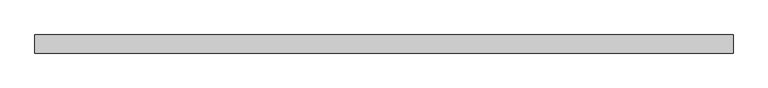
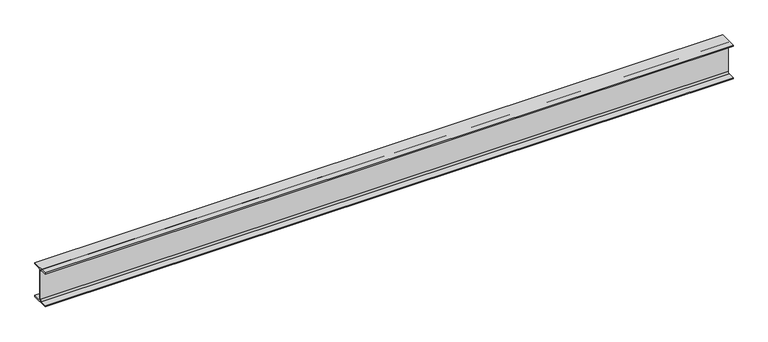
"""IFC4 building model written with IfcOpenShell, lengths in millimetres: beam geometry, 0912_Steel Framing_H-KSD3502 : H_SB_ASB_H-250x125x6x9."""

from ifc_helpers import new_model, si_unit, point, frame, frame_2d, origin, place, context, project, spatial, polyline, circle_curve, trimmed, segment, composite_curve, outline, extrude, source, transform, mapped, element, save


def beam_1a29c797(model_context):
    return source(origin(), model_context, "Body", "SweptSolid", [
        extrude(outline(composite_curve([segment(polyline([(62.5, -116.0), (62.5, -125.0), (-62.5, -125.0), (-62.5, -116.0), (-15.0, -116.0)]), True, "CONTINUOUS"), segment(trimmed(circle_curve(frame_2d((-15.0, -104.0)), 12.0), [point((-15.0, -116.0))], [point((-3.0, -104.0))], True, "CARTESIAN"), True, "CONTINUOUS"), segment(polyline([(-3.0, -104.0), (-3.0, 104.0)]), True, "CONTINUOUS"), segment(trimmed(circle_curve(frame_2d((-15.0, 104.0)), 12.0), [point((-3.0, 104.0))], [point((-15.0, 116.0))], True, "CARTESIAN"), True, "CONTINUOUS"), segment(polyline([(-15.0, 116.0), (-62.5, 116.0), (-62.5, 125.0), (62.5, 125.0), (62.5, 116.0), (15.0, 116.0)]), True, "CONTINUOUS"), segment(trimmed(circle_curve(frame_2d((15.0, 104.0)), 12.0), [point((15.0, 116.0))], [point((3.0, 104.0))], True, "CARTESIAN"), True, "CONTINUOUS"), segment(polyline([(3.0, 104.0), (3.0, -104.0)]), True, "CONTINUOUS"), segment(trimmed(circle_curve(frame_2d((15.0, -104.0)), 12.0), [point((3.0, -104.0))], [point((15.0, -116.0))], True, "CARTESIAN"), True, "CONTINUOUS"), segment(polyline([(15.0, -116.0), (62.5, -116.0)]), True, "CONTINUOUS")], self_intersect=False)), frame((-2404.8281705, 0.0, 0.0), z_axis=(1.0, 0.0, 0.0), x_axis=(0.0, 1.0, 0.0)), (0.0, 0.0, 1.0), 4808.1916513),
    ])


if __name__ == "__main__":
    model = new_model("IFC4")
    model_context = context("Model", 3, world=origin())
    ifc_project = project(units=[si_unit("LENGTHUNIT", "METRE", prefix="MILLI")], contexts=[model_context])
    site = spatial("IfcSite", under=ifc_project)
    building = spatial("IfcBuilding", under=site)
    placement = place(None, origin())
    beam_shape = beam_1a29c797(model_context)
    element("IfcBeam", 1, ObjectType="0912_Steel Framing_H-KSD3502 : H_SB_ASB_H-250x125x6x9", at=placement, inside=building, context=model_context, shape_type="MappedRepresentation", body=[
        mapped(beam_shape, transform((0.0, 0.0, 0.0), x_axis=(1.0, 0.0, 0.0), y_axis=(0.0, 1.0, 0.0), z_axis=(0.0, 0.0, 1.0))),
    ])
    save(model, "model.ifc")

# Revit data of these elements
# Type "0912_Steel Framing_H-KSD3502 : H_SB_ASB_H-250x125x6x9"
#   H_WM Code_1 = "S01AA003-00001 | Main Steel Structure Fabrication Work | Shelter/Building | Light Steel - Standard (30KG/M>Weight) | Material: (   )"
#   H_WM Code_2 = "S03AA029-00001 | Main Steel Structure Erection Work | Shelter/Building | Light Steel (30KG/M>Weight) | Material: (   )"
#   H_WM Code_3 = "S01AA010-00001 | Main Steel Structure Fabrication Work | Shelter/Building | Steel Painting/Coating | for Non-Fireproofed Steel Surface, Surface Preparation, Primer, Second & Final Coat | Material: (   )"
#   H_Q'ty Cal Type Tag = "SB-Q2"
#   Width = 12.5 cm
#   Web Thickness = 0.6 cm
#   Web Fillet = 1.2 cm
#   Warping Constant = 42539.8 cm⁶
#   W = 0
#   Torsional Moment of Inertia = 7.8102 cm⁴
#   Section Area = 37.66 cm²
#   Plastic Modulus weak axis = 73.1 cm³
#   Plastic Modulus strong axis = 366.0 cm³
#   Perimeter = 0.97 m²/m
#   Nominal Weight = 29.60 kgf/m
#   Moment of Inertia weak axis = 294.00 cm⁴
#   Moment of Inertia strong axis = 4050.00 cm⁴
#   Height = 25.0 cm
#   Flange Thickness = 0.9 cm
#   Elastic Modulus weak axis = 47.0 cm³
#   Elastic Modulus strong axis = 324.0 cm³
#   Centroid Vertical = 12.5 cm
#   Centroid Horizontal = 6.25 cm
#   Ix = 40500000
#   Length [instance default] = 1.5240 m
#   Zx = 366000
#   b = 0.1250 m
#   h = 0.2500 m
#   r = 0.0120 m
#   s = 0.0060 m
#   t = 0.0090 m
#   A = 0.003766 m²
#   Structural Material [instance default] = Steel, 45-345
#   Assembly Code = ""
# Element 1 (IfcBeam, "0912_Steel Framing_H-KSD3502 : H_SB_ASB_H-250x125x6x9")
#   Structural Material = none
# Materials
#   "Steel, 45-345": class "Metal", colour RGB 189 187 185, transparency 0, Description = "Steel 345 MPa", Cost = 0
